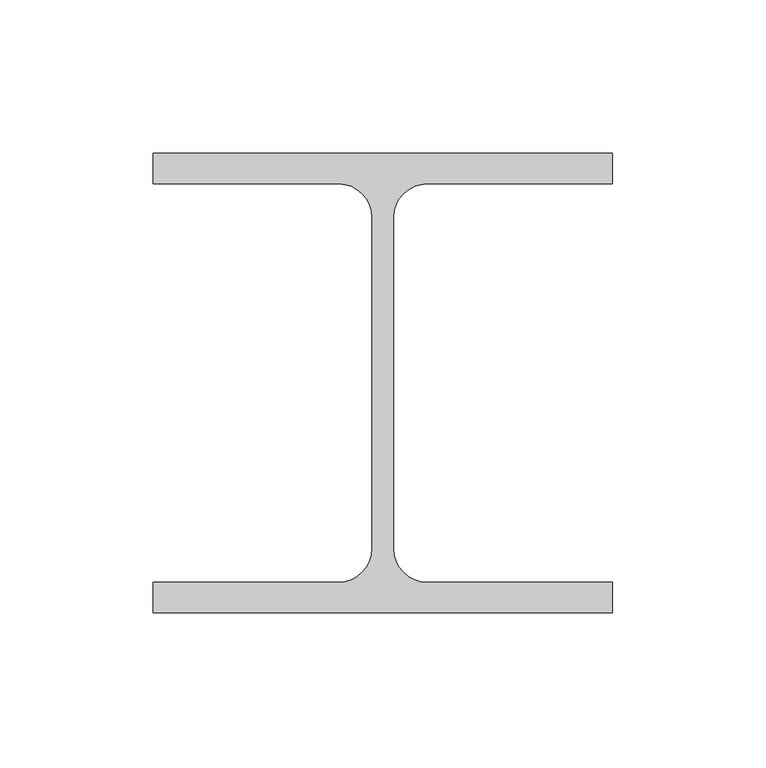
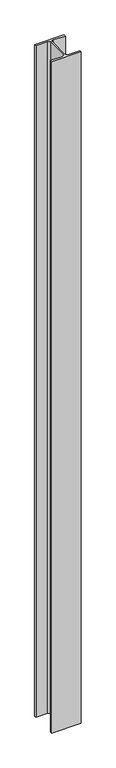
"""IFC4 building model written with IfcOpenShell, lengths in millimetres: column geometry, Steel Column_H_KSD3502 : H_SC_ASC_H-150x150x7x10."""

import ifcopenshell
import ifcopenshell.guid

model = None  # the IFC model being written
_history = None  # IfcOwnerHistory: only IFC2X3 demands one
_inside = {}  # id of a spatial element -> (the spatial element, [elements in it])
_under = {}  # id of a project, library or spatial element -> (it, [spatial elements below it])
_declared = {}  # id of a project -> (the project, [libraries it declares])
_typed = {}  # id of a type object -> (the type object, [elements of that type])
_made_of = {}  # id of a material, layer set ... -> (it, [elements and type objects made of it])


def new_model(schema):
    """Start an empty IFC model of exactly this schema.

    Asked for "IFC4X3", IfcOpenShell would pick the latest addendum, in which some entities
    have other attributes; the version numbers below select the first issue.
    IFC2X3 requires an IfcOwnerHistory on every rooted entity: one is made here for all.
    """
    global model, _history
    if schema == "IFC4X3":
        model = ifcopenshell.file(schema_version=(4, 3, 0, 0))
    else:
        model = ifcopenshell.file(schema=schema)
    _inside.clear()
    _under.clear()
    _declared.clear()
    _typed.clear()
    _made_of.clear()
    _history = None
    if model.schema == "IFC2X3":
        org = make("IfcOrganization", Name="unknown")
        user = make(
            "IfcPersonAndOrganization",
            ThePerson=make("IfcPerson", FamilyName="unknown"),
            TheOrganization=org,
        )
        app = make(
            "IfcApplication",
            ApplicationDeveloper=org,
            Version="unknown",
            ApplicationFullName="unknown",
            ApplicationIdentifier="unknown",
        )
        _history = make(
            "IfcOwnerHistory",
            OwningUser=user,
            OwningApplication=app,
            ChangeAction="ADDED",
            CreationDate=0,
        )
    return model


def make(cls, **values):
    """One entity of the class cls with the attributes given. An attribute that is None is left unset."""
    return model.create_entity(
        cls, **{name: value for name, value in values.items() if value is not None}
    )


def rooted(cls, **values):
    """An entity with a GlobalId (a new one), such as an element, a storey or a relation."""
    return make(cls, GlobalId=ifcopenshell.guid.new(), OwnerHistory=_history, **values)


def si_unit(unit_type, name, prefix=None):
    """IfcSIUnit, for example si_unit("LENGTHUNIT", "METRE", prefix="MILLI")."""
    return make("IfcSIUnit", UnitType=unit_type, Prefix=prefix, Name=name)


def assignment(units):
    """IfcUnitAssignment: the units of a project."""
    return None if units is None else make("IfcUnitAssignment", Units=units)


def point(xyz):
    """IfcCartesianPoint."""
    return None if xyz is None else make("IfcCartesianPoint", Coordinates=xyz)


def direction(xyz):
    """IfcDirection."""
    return None if xyz is None else make("IfcDirection", DirectionRatios=xyz)


def frame(location, z_axis=None, x_axis=None):
    """IfcAxis2Placement3D, a coordinate frame: its origin and axes. An axis left out is left unset."""
    return make(
        "IfcAxis2Placement3D",
        Location=point(location),
        Axis=direction(z_axis),
        RefDirection=direction(x_axis),
    )


def frame_2d(location, x_axis=None):
    """IfcAxis2Placement2D, a coordinate frame in the plane: its origin and x axis."""
    return make(
        "IfcAxis2Placement2D", Location=point(location), RefDirection=direction(x_axis)
    )


def origin():
    """The frame at (0, 0, 0) with its axes left unset."""
    return frame((0.0, 0.0, 0.0))


def place(relative_to, where):
    """IfcLocalPlacement: puts the frame where relative to a parent placement (None: the world)."""
    return make(
        "IfcLocalPlacement", PlacementRelTo=relative_to, RelativePlacement=where
    )


def context(
    kind, dimensions, precision=None, world=None, true_north=None, identifier=None
):
    """IfcGeometricRepresentationContext, for example the 3D "Model" context."""
    return make(
        "IfcGeometricRepresentationContext",
        ContextIdentifier=identifier,
        ContextType=kind,
        CoordinateSpaceDimension=dimensions,
        Precision=precision,
        WorldCoordinateSystem=world,
        TrueNorth=true_north,
    )


def project(units=None, contexts=None):
    """IfcProject with its units and contexts."""
    return rooted(
        "IfcProject",
        Name="project",
        RepresentationContexts=contexts,
        UnitsInContext=assignment(units),
    )


def spatial(cls, under=None, at=None, **own):
    """A site, building, storey or space (cls), placed at a placement, below another one or the project."""
    s = rooted(cls, ObjectPlacement=at, **own)
    if under is not None:
        _under.setdefault(under.id(), (under, []))[1].append(s)
    return s


def polyline(points):
    """IfcPolyline through the points."""
    return make("IfcPolyline", Points=[point(p) for p in points])


def circle_curve(where, radius):
    """IfcCircle in the frame where."""
    return make("IfcCircle", Position=where, Radius=radius)


def trimmed(basis, trim1, trim2, sense, master):
    """IfcTrimmedCurve: the piece of a basis curve between two trims."""
    return make(
        "IfcTrimmedCurve",
        BasisCurve=basis,
        Trim1=trim1,
        Trim2=trim2,
        SenseAgreement=sense,
        MasterRepresentation=master,
    )


def segment(curve, same_sense, transition):
    """IfcCompositeCurveSegment."""
    return make(
        "IfcCompositeCurveSegment",
        Transition=transition,
        SameSense=same_sense,
        ParentCurve=curve,
    )


def composite_curve(segments, self_intersect=None):
    """IfcCompositeCurve: segments joined end to end."""
    return make("IfcCompositeCurve", Segments=segments, SelfIntersect=self_intersect)


def outline(outer, holes=None, kind="AREA"):
    """IfcArbitraryClosedProfileDef: a profile drawn as a closed curve; with holes, ...WithVoids."""
    if holes is None:
        return make("IfcArbitraryClosedProfileDef", ProfileType=kind, OuterCurve=outer)
    return make(
        "IfcArbitraryProfileDefWithVoids",
        ProfileType=kind,
        OuterCurve=outer,
        InnerCurves=holes,
    )


def extrude(swept, where, along, depth):
    """IfcExtrudedAreaSolid: the profile swept, set in the frame where, extruded along a direction by depth."""
    return make(
        "IfcExtrudedAreaSolid",
        SweptArea=swept,
        Position=where,
        ExtrudedDirection=direction(along),
        Depth=depth,
    )


def shape(context_of_items, identifier, shape_type, items):
    """IfcShapeRepresentation: the items that make up one representation, for example the "Body"."""
    return make(
        "IfcShapeRepresentation",
        ContextOfItems=context_of_items,
        RepresentationIdentifier=identifier,
        RepresentationType=shape_type,
        Items=items,
    )


def source(mapping_origin, context_of_items, identifier, shape_type, items):
    """IfcRepresentationMap: a shape defined once, which mapped items show again and again."""
    return make(
        "IfcRepresentationMap",
        MappingOrigin=mapping_origin,
        MappedRepresentation=shape(context_of_items, identifier, shape_type, items),
    )


def transform(
    local_origin,
    x_axis=None,
    y_axis=None,
    z_axis=None,
    scale=None,
    scale2=None,
    scale3=None,
    uniform=True,
):
    """IfcCartesianTransformationOperator3D, or its non-uniform kind. x_axis, y_axis, z_axis: its Axis1, 2, 3."""
    if uniform:
        return make(
            "IfcCartesianTransformationOperator3D",
            Axis1=direction(x_axis),
            Axis2=direction(y_axis),
            LocalOrigin=point(local_origin),
            Scale=scale,
            Axis3=direction(z_axis),
        )
    return make(
        "IfcCartesianTransformationOperator3DnonUniform",
        Axis1=direction(x_axis),
        Axis2=direction(y_axis),
        LocalOrigin=point(local_origin),
        Scale=scale,
        Axis3=direction(z_axis),
        Scale2=scale2,
        Scale3=scale3,
    )


def mapped(mapping_source, mapping_target):
    """IfcMappedItem: shows the shape of a source again, moved by a transform."""
    return make(
        "IfcMappedItem", MappingSource=mapping_source, MappingTarget=mapping_target
    )


def made_of(thing, what):
    """Note that an element or type object is made of a material, layer set ...; save() writes the relation."""
    if what is not None:
        _made_of.setdefault(what.id(), (what, []))[1].append(thing)
    return thing


def element(
    cls,
    number,
    at=None,
    inside=None,
    cuts=None,
    type_object=None,
    material=None,
    context=None,
    identifier="Body",
    shape_type=None,
    held_by="IfcProductDefinitionShape",
    body=None,
    shapes=None,
    **own,
):
    """One element of the class cls, such as IfcWall. Its Tag is "e" and its number.

    at: its placement. inside: the storey or other place that contains it. cuts: it is an
    opening in that element (IfcRelVoidsElement). A single representation is given by context,
    identifier, shape_type and body (its items); several are given by shapes. held_by: the class
    of the entity that holds the representations. save() writes the other relations.
    """
    e = rooted(cls, Tag="e%d" % number, ObjectPlacement=at, **own)
    if body is not None:
        shapes = [shape(context, identifier, shape_type, body)]
    if shapes is not None:
        e.Representation = make(held_by, Representations=shapes)
    if inside is not None:
        _inside.setdefault(inside.id(), (inside, []))[1].append(e)
    if cuts is not None:
        rooted(
            "IfcRelVoidsElement", RelatingBuildingElement=cuts, RelatedOpeningElement=e
        )
    if type_object is not None:
        _typed.setdefault(type_object.id(), (type_object, []))[1].append(e)
    return made_of(e, material)


def aggregate(whole, parts):
    """IfcRelAggregates: a whole, such as a stair, and the parts it consists of."""
    return rooted("IfcRelAggregates", RelatingObject=whole, RelatedObjects=parts)


def save(model, path):
    """Write the relations noted so far, then the file.

    IfcRelAggregates (storeys below a building ...), IfcRelContainedInSpatialStructure (elements
    in a storey), IfcRelDefinesByType, IfcRelAssociatesMaterial and IfcRelDeclares: one each for
    every whole, place, type object, material and project.
    """
    for whole, parts in _under.values():
        aggregate(whole, parts)
    for where, things in _inside.values():
        rooted(
            "IfcRelContainedInSpatialStructure",
            RelatedElements=things,
            RelatingStructure=where,
        )
    for kind, things in _typed.values():
        rooted("IfcRelDefinesByType", RelatedObjects=things, RelatingType=kind)
    for what, things in _made_of.values():
        rooted("IfcRelAssociatesMaterial", RelatedObjects=things, RelatingMaterial=what)
    for by, libraries in _declared.values():
        rooted("IfcRelDeclares", RelatingContext=by, RelatedDefinitions=libraries)
    model.write(path)


def column_0d026061(model_context):
    return source(origin(), model_context, "Body", "SweptSolid", [
        extrude(outline(composite_curve([segment(polyline([(75.0, 75.0), (75.0, 65.0), (14.5, 65.0)]), True, "CONTINUOUS"), segment(trimmed(circle_curve(frame_2d((14.5, 54.0)), 11.0), [point((14.5, 65.0))], [point((3.5, 54.0))], True, "CARTESIAN"), True, "CONTINUOUS"), segment(polyline([(3.5, 54.0), (3.5, -54.0)]), True, "CONTINUOUS"), segment(trimmed(circle_curve(frame_2d((14.5, -54.0)), 11.0), [point((3.5, -54.0))], [point((14.5, -65.0))], True, "CARTESIAN"), True, "CONTINUOUS"), segment(polyline([(14.5, -65.0), (75.0, -65.0), (75.0, -75.0), (-75.0, -75.0), (-75.0, -65.0), (-14.5, -65.0)]), True, "CONTINUOUS"), segment(trimmed(circle_curve(frame_2d((-14.5, -54.0)), 11.0), [point((-14.5, -65.0))], [point((-3.5, -54.0))], True, "CARTESIAN"), True, "CONTINUOUS"), segment(polyline([(-3.5, -54.0), (-3.5, 54.0)]), True, "CONTINUOUS"), segment(trimmed(circle_curve(frame_2d((-14.5, 54.0)), 11.0), [point((-3.5, 54.0))], [point((-14.5, 65.0))], True, "CARTESIAN"), True, "CONTINUOUS"), segment(polyline([(-14.5, 65.0), (-75.0, 65.0), (-75.0, 75.0), (75.0, 75.0)]), True, "CONTINUOUS")], self_intersect=False)), frame((0.0, 0.0, 8299.9720055), z_axis=(0.0, 0.0, 1.0), x_axis=(1.0, 0.0, 0.0)), (0.0, 0.0, 1.0), 3610.0),
    ])


if __name__ == "__main__":
    model = new_model("IFC4")
    model_context = context("Model", 3, world=origin())
    ifc_project = project(units=[si_unit("LENGTHUNIT", "METRE", prefix="MILLI")], contexts=[model_context])
    site = spatial("IfcSite", under=ifc_project)
    building = spatial("IfcBuilding", under=site)
    placement = place(None, origin())
    column_shape = column_0d026061(model_context)
    element("IfcColumn", 1, ObjectType="Steel Column_H_KSD3502 : H_SC_ASC_H-150x150x7x10", at=placement, inside=building, context=model_context, shape_type="MappedRepresentation", body=[
        mapped(column_shape, transform((0.0, 0.0, 0.0), x_axis=(1.0, 0.0, 0.0), y_axis=(0.0, 1.0, 0.0), z_axis=(0.0, 0.0, 1.0))),
    ])
    save(model, "model.ifc")

# Revit data of these elements
# Type "Steel Column_H_KSD3502 : H_SC_ASC_H-150x150x7x10"
#   Width = 15.0 cm
#   Web Thickness = 0.7 cm
#   Web Fillet = 1.1 cm
#   Warping Constant = 27562.5 cm⁶
#   Torsional Moment of Inertia = 11.6007 cm⁴
#   Section Area = 40.14 cm²
#   Plastic Modulus weak axis = 115.0 cm³
#   Plastic Modulus strong axis = 246.0 cm³
#   Perimeter = 1.27 m²/m
#   Nominal Weight = 31.50 kgf/m
#   Moment of Inertia weak axis = 563.00 cm⁴
#   Moment of Inertia strong axis = 1640.00 cm⁴
#   Height = 15.0 cm
#   Flange Thickness = 1.0 cm
#   Elastic Modulus weak axis = 75.1 cm³
#   Elastic Modulus strong axis = 219.0 cm³
#   Centroid Vertical = 7.5 cm
#   Centroid Horizontal = 7.5 cm
#   Bolt Spacing = 13.97 cm
#   Structural Material [instance default] = Steel, 45-345
#   Section Name Key = ""
#   Assembly Code = ""
# Element 1 (IfcColumn, "Steel Column_H_KSD3502 : H_SC_ASC_H-150x150x7x10")
#   Structural Material = none
# Materials
#   "Steel, 45-345": class "Metal", colour RGB 189 187 185, transparency 0, Description = "Steel 345 MPa", Cost = 0
